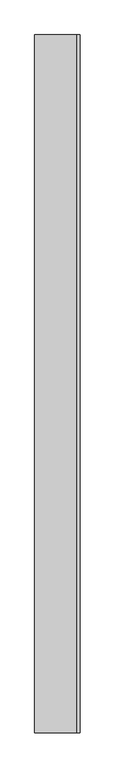
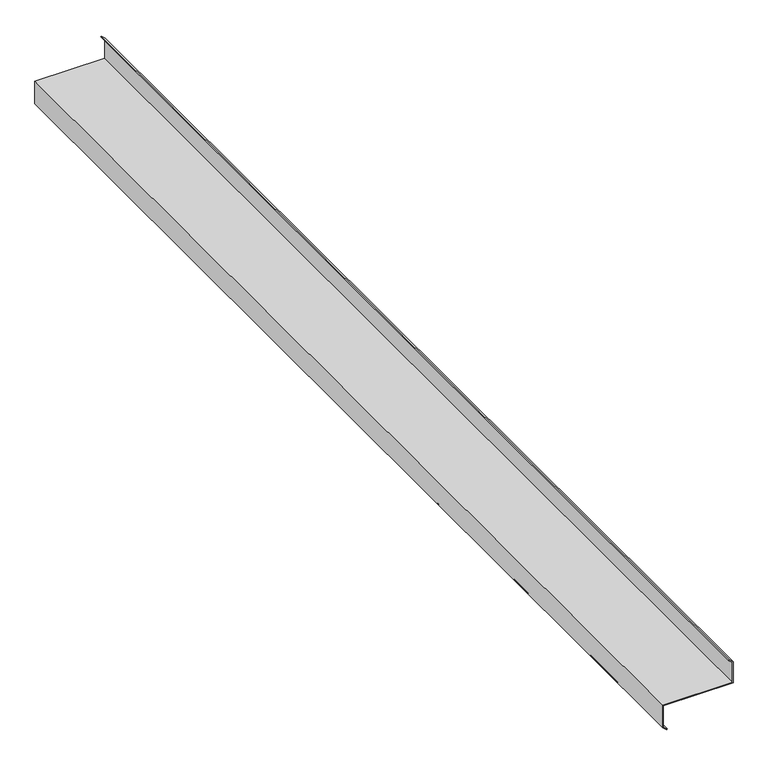
"""IFC4 building model written with IfcOpenShell, lengths in millimetres: proxy geometry, Generic Models 7:Generic Models 1:1:Generic Models 1:1 : Generic Models 7:Generic Models 1:337419:29 : Generic Models 7:Generic Models 1:1:Generic Models 1:1 : Generic Models 7:Generic Models 1:337419:306201."""

from ifc_helpers import new_model, si_unit, frame, origin, place, context, project, spatial, polyline, outline, extrude, source, transform, mapped, element, save


def generic_models_a6951b1f(model_context):
    return source(origin(), model_context, "Body", "SweptSolid", [
        extrude(outline(polyline([(1396.3591063, 667530.7466425), (1384.7904762, 667544.533599), (1309.4890623, 667544.533599), (1309.4890623, 667293.3117239), (1223.7640623, 667293.3117239), (1211.5189583, 667307.9048706), (1213.6471255, 667309.6906149), (1225.0595233, 667296.0898489), (1306.7109373, 667296.0898489), (1306.7109373, 667547.3117239), (1386.0859372, 667547.3117239), (1398.3310411, 667532.7185773), (1396.3591063, 667530.7466425)])), frame((0.0, -568533.14606, 0.0), z_axis=(0.0, 1.0, 0.0), x_axis=(0.0, 0.0, 1.0)), (0.0, 0.0, 1.0), 3924.7296759),
    ])


if __name__ == "__main__":
    model = new_model("IFC4")
    model_context = context("Model", 3, world=origin())
    ifc_project = project(units=[si_unit("LENGTHUNIT", "METRE", prefix="MILLI")], contexts=[model_context])
    site = spatial("IfcSite", under=ifc_project)
    building = spatial("IfcBuilding", under=site)
    placement = place(None, origin())
    generic_models_shape = generic_models_a6951b1f(model_context)
    element("IfcBuildingElementProxy", 1, Name="Generic Models 7:Generic Models 1:1:Generic Models 1:1 : Generic Models 7:Generic Models 1:337419:29 : Generic Models 7:Generic Models 1:1:Generic Models 1:1 : Generic Models 7:Generic Models 1:337419:306201", ObjectType="Generic Models 7:Generic Models 1:1:Generic Models 1:1 : Generic Models 7:Generic Models 1:337419:29 : Generic Models 7:Generic Models 1:1:Generic Models 1:1 : Generic Models 7:Generic Models 1:337419:306201", at=placement, inside=building, context=model_context, shape_type="MappedRepresentation", body=[
        mapped(generic_models_shape, transform((0.0, 0.0, 0.0), x_axis=(1.0, 0.0, 0.0), y_axis=(0.0, 1.0, 0.0), z_axis=(0.0, 0.0, 1.0))),
    ])
    save(model, "model.ifc")

# Revit data of these elements
# Type "Generic Models 7:Generic Models 1:1:Generic Models 1:1 : Generic Models 7:Generic Models 1:337419:29 : Generic Models 7:Generic Models 1:1:Generic Models 1:1 : Generic Models 7:Generic Models 1:337419:306201"
#   NameOverride = "Generic Models 7:Generic Models 1:1:Generic Models 1:1 : Generic Models 7:Generic Models 1:337419:306201"
#   ObjectTypeOverride = "Generic Models 1:1 : Generic Models 7:Generic Models 1:337419"
#   Reference = "Generic Models 1"
#   Tag = "306201"
# Element 1 (IfcBuildingElementProxy, "Generic Models 7:Generic Models 1:1:Generic Models 1:1 : Generic Models 7:Generic Models 1:337419:29 : Generic Models 7:Generic Models 1:1:Generic Models 1:1 : Generic Models 7:Generic Models 1:337419:306201")
#   Materials on its faces: "CEE' SECTION (8.0x3.5C - SEE STRUCT. DWGS)"
# Materials
#   "CEE' SECTION (8.0x3.5C - SEE STRUCT. DWGS)": class "Unassigned", colour RGB 210 209 208, transparency 0, Keynote = "M05121300.02", Cost = 0
